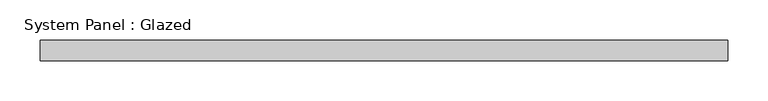
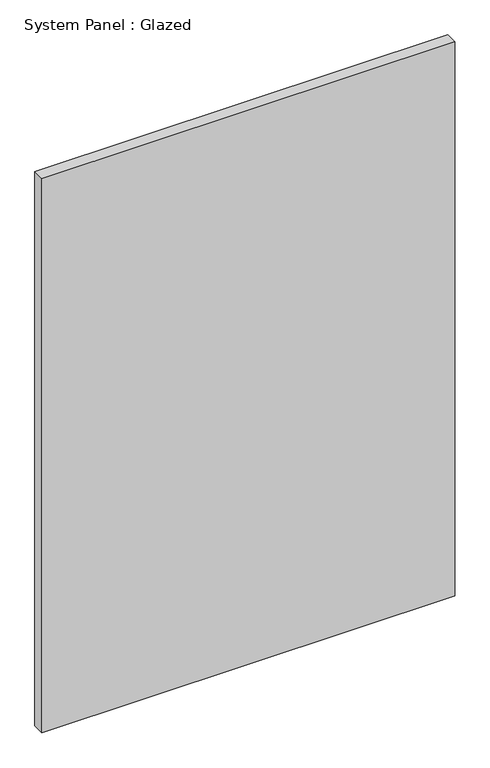
"""IFC4 building model written with IfcOpenShell, lengths in millimetres: plate geometry, System Panel : Glazed."""

from ifc_helpers import new_model, si_unit, origin, origin_with_axes, place, context, project, spatial, polyline, outline, extrude, source, transform, mapped, element, save


def system_panel_glazed_e397b593(model_context):
    return source(origin(), model_context, "Body", "SweptSolid", [
        extrude(outline(polyline([(427.9999998, 19.05), (-427.9999998, 19.05), (-427.9999998, 44.45), (427.9999998, 44.45), (427.9999998, 19.05)])), origin_with_axes(), (0.0, 0.0, 1.0), 1216.0),
    ])


if __name__ == "__main__":
    model = new_model("IFC4")
    model_context = context("Model", 3, world=origin())
    ifc_project = project(units=[si_unit("LENGTHUNIT", "METRE", prefix="MILLI")], contexts=[model_context])
    site = spatial("IfcSite", under=ifc_project)
    building = spatial("IfcBuilding", under=site)
    placement = place(None, origin())
    system_panel_glazed_shape = system_panel_glazed_e397b593(model_context)
    element("IfcPlate", 1, ObjectType="System Panel : Glazed", at=placement, inside=building, context=model_context, shape_type="MappedRepresentation", body=[
        mapped(system_panel_glazed_shape, transform((0.0, 0.0, 0.0), x_axis=(1.0, 0.0, 0.0), y_axis=(0.0, 1.0, 0.0), z_axis=(0.0, 0.0, 1.0))),
    ])
    save(model, "model.ifc")

# Revit data of these elements
# Type "System Panel : Glazed"
#   Construction Type Id = "GSP4R"
#   Analytic Construction = "1/8 in Pilkington single glazing"
#   Visual Light Transmittance = 0.9
#   Solar Heat Gain Coefficient = 0.86
#   Heat Transfer Coefficient (U) = 6.7069 W/(m²·K)
# Element 1 (IfcPlate, "System Panel : Glazed")
#   Materials on its faces: "Glass"
# Materials
#   "Glass": class "Glass", colour RGB 0 128 192, transparency 0.75, Description = "Soda Lime Glass", Cost = 0
